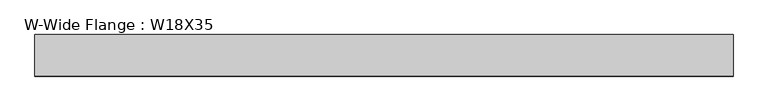
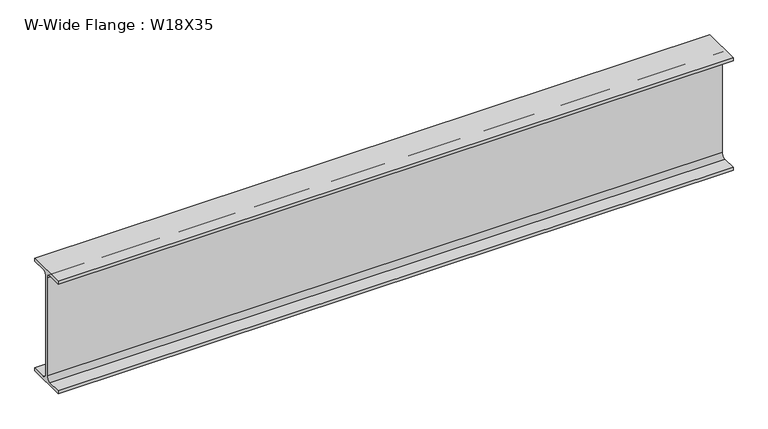
"""IFC4 building model written with IfcOpenShell, lengths in millimetres: beam geometry, W-Wide Flange : W18X35."""

from ifc_helpers import new_model, si_unit, point, frame, frame_2d, origin, place, context, project, spatial, polyline, circle_curve, trimmed, segment, composite_curve, outline, extrude, source, transform, mapped, element, save


def w_wide_flange_w18x35_99f9f71b(model_context):
    return source(origin(), model_context, "Body", "SweptSolid", [
        extrude(outline(composite_curve([segment(polyline([(76.2, -213.995), (76.2, -224.79), (-76.2, -224.79), (-76.2, -213.995), (-21.59, -213.995)]), True, "CONTINUOUS"), segment(trimmed(circle_curve(frame_2d((-21.59, -196.215)), 17.78), [point((-21.59, -213.995))], [point((-3.81, -196.215))], True, "CARTESIAN"), True, "CONTINUOUS"), segment(polyline([(-3.81, -196.215), (-3.81, 196.215)]), True, "CONTINUOUS"), segment(trimmed(circle_curve(frame_2d((-21.59, 196.215)), 17.78), [point((-3.81, 196.215))], [point((-21.59, 213.995))], True, "CARTESIAN"), True, "CONTINUOUS"), segment(polyline([(-21.59, 213.995), (-76.2, 213.995), (-76.2, 224.79), (76.2, 224.79), (76.2, 213.995), (21.59, 213.995)]), True, "CONTINUOUS"), segment(trimmed(circle_curve(frame_2d((21.59, 196.215)), 17.78), [point((21.59, 213.995))], [point((3.81, 196.215))], True, "CARTESIAN"), True, "CONTINUOUS"), segment(polyline([(3.81, 196.215), (3.81, -196.215)]), True, "CONTINUOUS"), segment(trimmed(circle_curve(frame_2d((21.59, -196.215)), 17.78), [point((3.81, -196.215))], [point((21.59, -213.995))], True, "CARTESIAN"), True, "CONTINUOUS"), segment(polyline([(21.59, -213.995), (76.2, -213.995)]), True, "CONTINUOUS")], self_intersect=False)), frame((-1279.525, 0.0, 0.0), z_axis=(1.0, 0.0, 0.0), x_axis=(0.0, 1.0, 0.0)), (0.0, 0.0, 1.0), 2559.05),
    ])


if __name__ == "__main__":
    model = new_model("IFC4")
    model_context = context("Model", 3, world=origin())
    ifc_project = project(units=[si_unit("LENGTHUNIT", "METRE", prefix="MILLI")], contexts=[model_context])
    site = spatial("IfcSite", under=ifc_project)
    building = spatial("IfcBuilding", under=site)
    placement = place(None, origin())
    w_wide_flange_w18x35_shape = w_wide_flange_w18x35_99f9f71b(model_context)
    element("IfcBeam", 1, ObjectType="W-Wide Flange : W18X35", at=placement, inside=building, context=model_context, shape_type="MappedRepresentation", body=[
        mapped(w_wide_flange_w18x35_shape, transform((0.0, 0.0, 0.0), x_axis=(1.0, 0.0, 0.0), y_axis=(0.0, 1.0, 0.0), z_axis=(0.0, 0.0, 1.0))),
    ])
    save(model, "model.ifc")

# Revit data of these elements
# Type "W-Wide Flange : W18X35"
#   Assembly Code = "B10"
#   W = 35
#   Length [instance default] = 5' - 0"
#   bf = 0' - 6"
#   d = 1' - 5.7"
#   k = 0' - 1 1/8"
#   k2 = 0' - 0.7"
#   tf = 0' - 0.425"
#   tw = 0' - 0.3"
#   A = 0.0715278 SF
#   Structural Material [instance default] = Steel ASTM A992
# Element 1 (IfcBeam, "W-Wide Flange : W18X35")
#   Structural Material = Steel ASTM A36
#   Materials on its faces: "Steel ASTM A36"
# Materials
#   "Steel ASTM A992": class "Metal", colour RGB 199 199 199, transparency 0, Description = "Structural steel 50ksi", Cost = 0
#   "Steel ASTM A36": class "Metal", colour RGB 199 199 199, transparency 0, Description = "Structural steel, ASTM A36 Grade B, mill finish", Cost = 0
